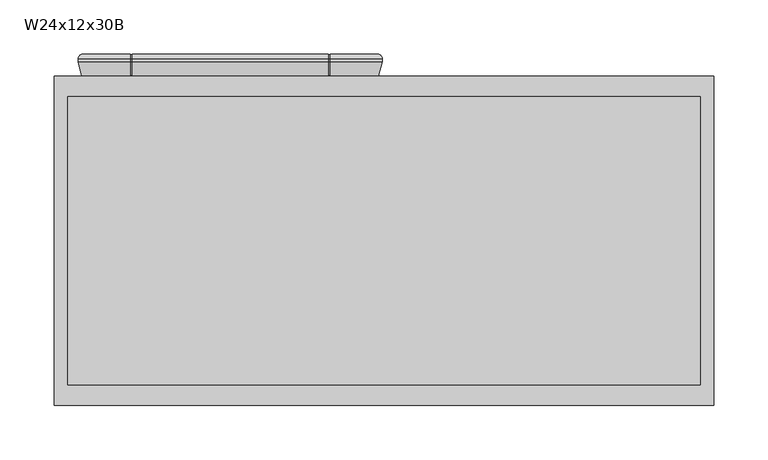
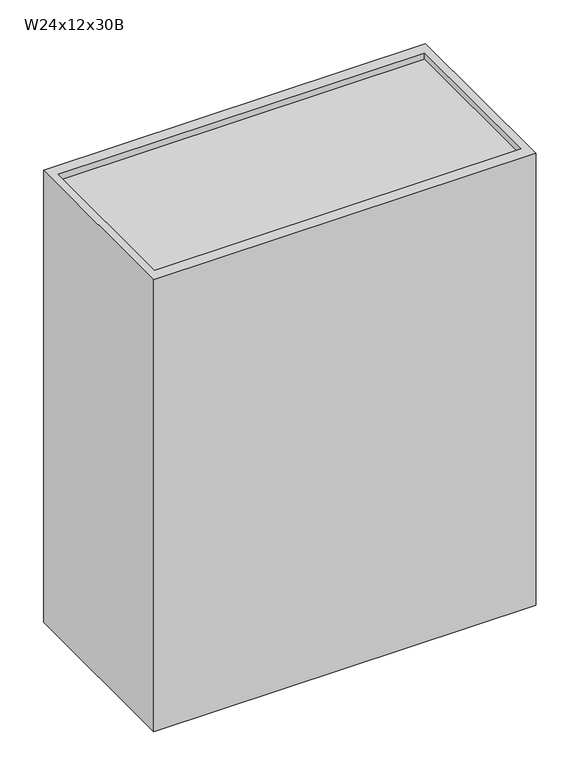
"""IFC4 building model written with IfcOpenShell, lengths in millimetres: furniture geometry, Cabinet-Wall-Merillat-Double_Door-Marlin : W24x12x30B."""

from ifc_helpers import new_model, si_unit, frame, origin, place, context, project, spatial, polyline, circle_curve, ellipse_curve, outline, extrude, faceted_brep, source, transform, mapped, element, save
from ifc_brep_helpers import plane_surface, cylinder_surface, advanced_brep


def w24x12x30b_f3964ec6(model_context):
    return source(origin(), model_context, "Body", "SolidModel", [
        advanced_brep(
        [(-24.0971608, 382.5621, 2108.2), (-21.0006683, 387.0325, 2105.1035075), (-21.0006683, 387.0325, 1400.0964925), (-24.0971608, 382.5621, 1397.0), (-24.0971608, 379.7935, 1397.0), (-24.0971608, 379.7935, 2108.2), (-20.5919608, 366.7125, 1400.5052), (-20.5919608, 366.7125, 2104.6948), (24.104002, 366.7125, 2059.9988372), (24.104002, 366.7125, 1445.2011628), (24.4741337, 367.50625, 1445.5712945), (26.5552927, 371.96931, 1447.6524535), (26.5552927, 371.96931, 2057.5475465), (24.4741337, 367.50625, 2059.6287055), (25.1555233, 374.2094093, 1446.252684), (25.1555233, 374.2094093, 2058.947316), (10.8278392, 374.4595, 1431.925), (10.8278392, 374.4595, 2073.275), (10.8278392, 379.2855, 1431.925), (10.8278392, 379.2855, 2073.275), (25.1555233, 379.5355907, 1446.252684), (25.1555233, 379.5355907, 2058.947316), (26.5552927, 381.77569, 1447.6524535), (26.5552927, 381.77569, 2057.5475465), (24.4741337, 386.23875, 1445.5712945), (24.1068694, 387.0263508, 1445.2040302), (24.104002, 387.0325, 2059.9988372), (24.4741337, 386.23875, 2059.6287055), (24.1068694, 387.0325, 1400.0964925), (24.1068694, 382.5621, 1397.0), (253.7938467, 387.0325, 1400.0964925), (256.8903392, 382.5621, 1397.0), (208.7261206, 382.5621, 1397.0), (208.7261206, 387.0325, 1400.0964925), (25.6943694, 382.5621, 1397.0), (25.6943694, 387.0325, 1400.0964925), (207.1386206, 387.0325, 1400.0964925), (207.1386206, 382.5621, 1397.0), (24.1068694, 379.7935, 1397.0), (256.8903392, 379.7935, 1397.0), (208.7261206, 379.7935, 1397.0), (25.6943694, 379.7935, 1397.0), (207.1386206, 379.7935, 1397.0), (24.1068694, 366.7125, 1400.5052), (253.3851392, 366.7125, 1400.5052), (208.7261206, 366.7125, 1400.5052), (25.6943694, 366.7125, 1400.5052), (207.1386206, 366.7125, 1400.5052), (206.2378857, 371.96931, 1447.6524535), (25.6943694, 367.50625, 1445.5712945), (25.6943694, 366.7125, 1445.2011628), (207.1386206, 366.7125, 1445.2011628), (207.1386206, 367.50625, 1445.5712945), (208.3190448, 367.50625, 1445.5712945), (207.6376552, 374.2094093, 1446.252684), (221.9653392, 374.4595, 1431.925), (221.9653392, 379.2855, 1431.925), (207.6376552, 379.5355907, 1446.252684), (206.2378857, 381.77569, 1447.6524535), (208.3190448, 386.23875, 1445.5712945), (207.1386206, 386.23875, 1445.5712945), (207.1386206, 387.0325, 1445.2011628), (25.6943694, 387.0325, 1445.2011628), (25.6943694, 386.23875, 1445.5712945), (253.7938467, 387.0325, 2105.1035075), (256.8903392, 382.5621, 2108.2), (256.8903392, 379.7935, 2108.2), (253.3851392, 366.7125, 2104.6948), (208.6891765, 366.7125, 1445.2011628), (208.6891765, 366.7125, 2059.9988372), (208.3190448, 367.50625, 2059.6287055), (206.2378857, 371.96931, 2057.5475465), (207.6376552, 374.2094093, 2058.947316), (221.9653392, 374.4595, 2073.275), (221.9653392, 379.2855, 2073.275), (207.6376552, 379.5355907, 2058.947316), (206.2378857, 381.77569, 2057.5475465), (208.3190448, 386.23875, 2059.6287055), (208.6891765, 387.0325, 2059.9988372), (208.6891765, 387.0325, 1445.2011628), (208.7261206, 387.0325, 2105.1035075), (208.7261206, 382.5621, 2108.2), (24.1068694, 382.5621, 2108.2), (24.1068694, 387.0325, 2105.1035075), (207.1386206, 382.5621, 2108.2), (207.1386206, 387.0325, 2105.1035075), (25.6943694, 387.0325, 2105.1035075), (25.6943694, 382.5621, 2108.2), (208.7261206, 379.7935, 2108.2), (24.1068694, 379.7935, 2108.2), (207.1386206, 379.7935, 2108.2), (25.6943694, 379.7935, 2108.2), (208.7261206, 366.7125, 2104.6948), (24.1068694, 366.7125, 2104.6948), (207.1386206, 366.7125, 2104.6948), (25.6943694, 366.7125, 2104.6948), (207.1386206, 366.7125, 2059.9988372), (25.6943694, 366.7125, 2059.9988372), (207.1386206, 367.50625, 2059.6287055), (25.6943694, 367.50625, 2059.6287055), (25.6943694, 386.23875, 2059.6287055), (25.6943694, 387.0325, 2059.9988372), (207.1386206, 387.0325, 2059.9988372), (207.1386206, 386.23875, 2059.6287055), (207.1386206, 367.50625, 2104.0857412), (207.1386206, 379.8980037, 2107.40625), (207.1386206, 382.5621, 2107.40625), (207.1386206, 386.23875, 2104.9526052), (208.7261206, 386.23875, 2059.6287055), (208.7261206, 386.23875, 2104.9526052), (208.7261206, 382.5621, 2107.40625), (208.7261206, 379.8980037, 2107.40625), (208.7261206, 367.50625, 2104.0857412), (208.7261206, 367.50625, 2059.6287055), (24.1068694, 367.50625, 2059.6287055), (24.1068694, 367.50625, 2104.0857412), (24.1068694, 379.8980037, 2107.40625), (24.1068694, 382.5621, 2107.40625), (24.1068694, 386.23875, 2104.9526052), (24.1068694, 386.23875, 2059.6287055), (25.6943694, 386.23875, 2104.9526052), (25.6943694, 382.5621, 2107.40625), (25.6943694, 379.8980037, 2107.40625), (25.6943694, 367.50625, 2104.0857412), (24.1068694, 386.23875, 1445.5712945), (24.1068694, 386.23875, 1400.2473948), (24.1068694, 382.5621, 1397.79375), (24.1068694, 379.8980037, 1397.79375), (24.1068694, 367.50625, 1401.1142588), (24.1068694, 367.50625, 1445.5712945), (25.6943694, 367.50625, 1401.1142588), (25.6943694, 379.8980037, 1397.79375), (25.6943694, 382.5621, 1397.79375), (25.6943694, 386.23875, 1400.2473948), (207.1386206, 386.23875, 1400.2473948), (207.1386206, 382.5621, 1397.79375), (207.1386206, 379.8980037, 1397.79375), (207.1386206, 367.50625, 1401.1142588), (208.7261206, 386.23875, 1445.5712945), (208.7261206, 367.50625, 1445.5712945), (208.7261206, 367.50625, 1401.1142588), (208.7261206, 379.8980037, 1397.79375), (208.7261206, 382.5621, 1397.79375), (208.7261206, 386.23875, 1400.2473948)],
        [
            (0, 1, ellipse_curve(frame((-19.3219608, 382.5621, 2103.4248), z_axis=(-0.7071067811865475, 0.0, -0.7071067811865475), x_axis=(-0.7071067811865474, 0.0, 0.7071067811865476)), 6.7531526, 4.7752)),
            (1, 2),
            (2, 3, ellipse_curve(frame((-19.3219608, 382.5621, 1401.7752), z_axis=(-0.7071067811865475, 0.0, 0.7071067811865475), x_axis=(0.7071067811865474, 0.0, 0.7071067811865476)), 6.7531526, 4.7752)),
            (3, 0),
            (3, 4),
            (4, 5),
            (5, 0),
            (4, 6),
            (6, 7),
            (7, 5),
            (8, 9),
            (9, 10),
            (10, 11),
            (11, 12),
            (12, 13),
            (13, 8),
            (11, 14, ellipse_curve(frame((25.1280392, 372.6348492, 1446.2252), z_axis=(-0.7071067811865475, 0.0, 0.7071067811865475), x_axis=(0.7071067811865474, 0.0, 0.7071067811865476)), 2.2271035, 1.5748)),
            (14, 15),
            (15, 12, ellipse_curve(frame((25.1280392, 372.6348492, 2058.9748), z_axis=(-0.7071067811865475, 0.0, -0.7071067811865475), x_axis=(-0.7071067811865474, 0.0, 0.7071067811865476)), 2.2271035, 1.5748)),
            (14, 16),
            (16, 17),
            (17, 15),
            (16, 18),
            (18, 19),
            (19, 17),
            (18, 20),
            (20, 21),
            (21, 19),
            (20, 22, ellipse_curve(frame((25.1280392, 381.1101508, 1446.2252), z_axis=(-0.7071067811865475, 0.0, 0.7071067811865475), x_axis=(0.7071067811865474, 0.0, 0.7071067811865476)), 2.2271035, 1.5748)),
            (22, 23),
            (23, 21, ellipse_curve(frame((25.1280392, 381.1101508, 2058.9748), z_axis=(-0.7071067811865475, 0.0, -0.7071067811865475), x_axis=(-0.7071067811865474, 0.0, 0.7071067811865476)), 2.2271035, 1.5748)),
            (22, 24),
            (24, 25),
            (25, 26),
            (26, 27),
            (27, 23),
            (2, 28),
            (28, 29, circle_curve(frame((24.1068694, 382.5621, 1401.7752), z_axis=(-1.0, 0.0, 0.0), x_axis=(0.0, -1.0, 0.0)), 4.7752)),
            (29, 3),
            (30, 31, ellipse_curve(frame((252.1151392, 382.5621, 1401.7752), z_axis=(-0.7071067811865475, 0.0, -0.7071067811865475), x_axis=(-0.7071067811865476, 0.0, 0.7071067811865474)), 6.7531526, 4.7752)),
            (31, 32),
            (32, 33, circle_curve(frame((208.7261206, 382.5621, 1401.7752), z_axis=(1.0, 0.0, 0.0), x_axis=(0.0, -1.0, 0.0)), 4.7752)),
            (33, 30),
            (34, 35, circle_curve(frame((25.6943694, 382.5621, 1401.7752), z_axis=(1.0, 0.0, 0.0), x_axis=(0.0, -1.0, 0.0)), 4.7752)),
            (35, 36),
            (36, 37, circle_curve(frame((207.1386206, 382.5621, 1401.7752), z_axis=(-1.0, 0.0, 0.0), x_axis=(0.0, -1.0, 0.0)), 4.7752)),
            (37, 34),
            (29, 38),
            (38, 4),
            (31, 39),
            (39, 40),
            (40, 32),
            (41, 34),
            (37, 42),
            (42, 41),
            (38, 43),
            (43, 6),
            (39, 44),
            (44, 45),
            (45, 40),
            (46, 41),
            (42, 47),
            (47, 46),
            (48, 11),
            (10, 49),
            (49, 50),
            (50, 51),
            (51, 52),
            (52, 53),
            (53, 48),
            (48, 54, ellipse_curve(frame((207.6651392, 372.6348492, 1446.2252), z_axis=(-0.7071067811865475, 0.0, -0.7071067811865475), x_axis=(-0.7071067811865476, 0.0, 0.7071067811865474)), 2.2271035, 1.5748)),
            (54, 14),
            (54, 55),
            (55, 16),
            (55, 56),
            (56, 18),
            (56, 57),
            (57, 20),
            (57, 58, ellipse_curve(frame((207.6651392, 381.1101508, 1446.2252), z_axis=(-0.7071067811865475, 0.0, -0.7071067811865475), x_axis=(-0.7071067811865476, 0.0, 0.7071067811865474)), 2.2271035, 1.5748)),
            (58, 22),
            (58, 59),
            (59, 60),
            (60, 61),
            (61, 62),
            (62, 63),
            (63, 24),
            (30, 64),
            (64, 65, ellipse_curve(frame((252.1151392, 382.5621, 2103.4248), z_axis=(0.7071067811865475, 0.0, -0.7071067811865475), x_axis=(-0.7071067811865474, 0.0, -0.7071067811865476)), 6.7531526, 4.7752)),
            (65, 31),
            (65, 66),
            (66, 39),
            (66, 67),
            (67, 44),
            (68, 69),
            (69, 70),
            (70, 71),
            (71, 48),
            (53, 68),
            (71, 72, ellipse_curve(frame((207.6651392, 372.6348492, 2058.9748), z_axis=(0.7071067811865475, 0.0, -0.7071067811865475), x_axis=(-0.7071067811865474, 0.0, -0.7071067811865476)), 2.2271035, 1.5748)),
            (72, 54),
            (72, 73),
            (73, 55),
            (73, 74),
            (74, 56),
            (74, 75),
            (75, 57),
            (75, 76, ellipse_curve(frame((207.6651392, 381.1101508, 2058.9748), z_axis=(0.7071067811865475, 0.0, -0.7071067811865475), x_axis=(-0.7071067811865474, 0.0, -0.7071067811865476)), 2.2271035, 1.5748)),
            (76, 58),
            (76, 77),
            (77, 78),
            (78, 79),
            (79, 59),
            (64, 80),
            (80, 81, circle_curve(frame((208.7261206, 382.5621, 2103.4248), z_axis=(1.0, 0.0, 0.0), x_axis=(0.0, -1.0, 0.0)), 4.7752)),
            (81, 65),
            (0, 82),
            (82, 83, circle_curve(frame((24.1068694, 382.5621, 2103.4248), z_axis=(-1.0, 0.0, 0.0), x_axis=(0.0, -1.0, 0.0)), 4.7752)),
            (83, 1),
            (84, 85, circle_curve(frame((207.1386206, 382.5621, 2103.4248), z_axis=(-1.0, 0.0, 0.0), x_axis=(0.0, -1.0, 0.0)), 4.7752)),
            (85, 86),
            (86, 87, circle_curve(frame((25.6943694, 382.5621, 2103.4248), z_axis=(1.0, 0.0, 0.0), x_axis=(0.0, -1.0, 0.0)), 4.7752)),
            (87, 84),
            (81, 88),
            (88, 66),
            (5, 89),
            (89, 82),
            (90, 84),
            (87, 91),
            (91, 90),
            (88, 92),
            (92, 67),
            (7, 93),
            (93, 89),
            (94, 90),
            (91, 95),
            (95, 94),
            (43, 9),
            (8, 93),
            (92, 69),
            (68, 45),
            (96, 94),
            (95, 97),
            (97, 96),
            (50, 46),
            (47, 51),
            (12, 71),
            (70, 98),
            (98, 96),
            (97, 99),
            (99, 13),
            (15, 72),
            (17, 73),
            (19, 74),
            (21, 75),
            (23, 76),
            (27, 100),
            (100, 101),
            (101, 102),
            (102, 103),
            (103, 77),
            (83, 26),
            (25, 28),
            (33, 79),
            (78, 80),
            (85, 102),
            (101, 86),
            (35, 62),
            (61, 36),
            (98, 104),
            (104, 105),
            (105, 106),
            (106, 107, circle_curve(frame((207.1386206, 382.5621, 2103.4248), z_axis=(-1.0, 0.0, 0.0), x_axis=(0.0, 0.0, 1.0)), 3.98145)),
            (107, 103),
            (78, 108),
            (108, 109),
            (109, 110, circle_curve(frame((208.7261206, 382.5621, 2103.4248), z_axis=(1.0, 0.0, 0.0), x_axis=(0.0, 0.0, 1.0)), 3.98145)),
            (110, 111),
            (111, 112),
            (112, 113),
            (113, 69),
            (77, 108),
            (107, 109),
            (106, 110),
            (105, 111),
            (104, 112),
            (70, 113),
            (8, 114),
            (114, 115),
            (115, 116),
            (116, 117),
            (117, 118, circle_curve(frame((24.1068694, 382.5621, 2103.4248), z_axis=(-1.0, 0.0, 0.0), x_axis=(0.0, 0.0, 1.0)), 3.98145)),
            (118, 119),
            (119, 26),
            (100, 120),
            (120, 121, circle_curve(frame((25.6943694, 382.5621, 2103.4248), z_axis=(1.0, 0.0, 0.0), x_axis=(0.0, 0.0, 1.0)), 3.98145)),
            (121, 122),
            (122, 123),
            (123, 99),
            (119, 27),
            (118, 120),
            (117, 121),
            (116, 122),
            (115, 123),
            (114, 13),
            (25, 124),
            (124, 125),
            (125, 126, circle_curve(frame((24.1068694, 382.5621, 1401.7752), z_axis=(-1.0, 0.0, 0.0), x_axis=(0.0, 0.0, 1.0)), 3.98145)),
            (126, 127),
            (127, 128),
            (128, 129),
            (129, 9),
            (49, 130),
            (130, 131),
            (131, 132),
            (132, 133, circle_curve(frame((25.6943694, 382.5621, 1401.7752), z_axis=(1.0, 0.0, 0.0), x_axis=(0.0, 0.0, 1.0)), 3.98145)),
            (133, 63),
            (129, 10),
            (128, 130),
            (127, 131),
            (126, 132),
            (125, 133),
            (124, 24),
            (60, 134),
            (134, 135, circle_curve(frame((207.1386206, 382.5621, 1401.7752), z_axis=(-1.0, 0.0, 0.0), x_axis=(0.0, 0.0, 1.0)), 3.98145)),
            (135, 136),
            (136, 137),
            (137, 52),
            (138, 79),
            (68, 139),
            (139, 140),
            (140, 141),
            (141, 142),
            (142, 143, circle_curve(frame((208.7261206, 382.5621, 1401.7752), z_axis=(1.0, 0.0, 0.0), x_axis=(0.0, 0.0, 1.0)), 3.98145)),
            (143, 138),
            (138, 59),
            (53, 139),
            (137, 140),
            (136, 141),
            (135, 142),
            (134, 143),
        ],
        [
            cylinder_surface(frame((-19.3219608, 382.5621, 2108.2), z_axis=(0.0, 0.0, 1.0), x_axis=(0.0, -1.0, 0.0)), 4.7752),
            plane_surface(frame((-24.0971608, 382.5621, 2108.2), z_axis=(-1.0, 0.0, 0.0), x_axis=(0.0, 0.0, -1.0))),
            plane_surface(frame((-24.0971608, 379.7935, 2108.2), z_axis=(-0.9659229350723619, -0.25882983502910506, 0.0), x_axis=(0.0, 0.0, -1.0))),
            plane_surface(frame((24.104002, 366.7125, 2059.9988372), z_axis=(0.9063077870366099, -0.4226182617407856, 0.0), x_axis=(0.0, 0.0, -1.0))),
            cylinder_surface(frame((25.1280392, 372.6348492, 2108.2), z_axis=(0.0, 0.0, 1.0000000000000002), x_axis=(0.01745240643729364, 0.9998476951563912, 0.0)), 1.5748),
            plane_surface(frame((25.1555233, 374.2094093, 2058.947316), z_axis=(0.017452406437322144, 0.9998476951563906, 0.0), x_axis=(0.0, 0.0, -1.0))),
            plane_surface(frame((10.8278392, 374.4595, 2073.275), z_axis=(1.0, 0.0, 0.0), x_axis=(0.0, 0.0, -1.0))),
            plane_surface(frame((10.8278392, 379.2855, 2073.275), z_axis=(0.01745240643727848, -0.9998476951563914, 0.0), x_axis=(0.0, 0.0, -1.0))),
            cylinder_surface(frame((25.1280392, 381.1101508, 2108.2), z_axis=(0.0, 0.0, 1.0000000000000002), x_axis=(0.9063077870367326, 0.42261826174052236, 0.0)), 1.5748),
            plane_surface(frame((26.5552927, 381.77569, 2057.5475465), z_axis=(0.9063077870366333, 0.4226182617407352, 0.0), x_axis=(0.0, 0.0, -1.0))),
            cylinder_surface(frame((-24.0971608, 382.5621, 1401.7752), z_axis=(-1.0, 0.0, 0.0), x_axis=(0.0, -1.0, 0.0)), 4.7752),
            plane_surface(frame((-24.0971608, 382.5621, 1397.0), z_axis=(0.0, 0.0, -1.0), x_axis=(1.0, 0.0, 0.0))),
            plane_surface(frame((-24.0971608, 379.7935, 1397.0), z_axis=(0.0, -0.2588298350291095, -0.9659229350723607), x_axis=(1.0, 0.0, 0.0))),
            plane_surface(frame((24.104002, 366.7125, 1445.2011628), z_axis=(0.0, -0.42261826174078143, 0.9063077870366119), x_axis=(1.0, 0.0, 0.0))),
            cylinder_surface(frame((-24.0971608, 372.6348492, 1446.2252), z_axis=(-1.0000000000000002, 0.0, 0.0), x_axis=(0.0, 0.9998476951563913, 0.017452406437289025)), 1.5748),
            plane_surface(frame((25.1555233, 374.2094093, 1446.252684), z_axis=(0.0, 0.9998476951563907, 0.01745240643731753), x_axis=(1.0, 0.0, 0.0))),
            plane_surface(frame((10.8278392, 374.4595, 1431.925), z_axis=(0.0, 0.0, 1.0), x_axis=(1.0, 0.0, 0.0))),
            plane_surface(frame((10.8278392, 379.2855, 1431.925), z_axis=(0.0, -0.9998476951563913, 0.017452406437283095), x_axis=(1.0, 0.0, 0.0))),
            cylinder_surface(frame((-24.0971608, 381.1101508, 1446.2252), z_axis=(-1.0000000000000002, 0.0, 0.0), x_axis=(0.0, 0.4226182617405265, 0.9063077870367306)), 1.5748),
            plane_surface(frame((26.5552927, 381.77569, 1447.6524535), z_axis=(0.0, 0.4226182617407394, 0.9063077870366314), x_axis=(1.0, 0.0, 0.0))),
            cylinder_surface(frame((252.1151392, 382.5621, 1397.0), z_axis=(0.0, 0.0, -1.0), x_axis=(0.0, -1.0, 0.0)), 4.7752),
            plane_surface(frame((256.8903392, 382.5621, 1397.0), z_axis=(1.0, 0.0, 0.0), x_axis=(0.0, 0.0, 1.0))),
            plane_surface(frame((256.8903392, 379.7935, 1397.0), z_axis=(0.9659229350723619, -0.25882983502910506, 0.0), x_axis=(0.0, 0.0, 1.0))),
            plane_surface(frame((208.6891765, 366.7125, 1445.2011628), z_axis=(-0.9063077870366099, -0.4226182617407856, 0.0), x_axis=(0.0, 0.0, 1.0))),
            cylinder_surface(frame((207.6651392, 372.6348492, 1397.0), z_axis=(0.0, 0.0, -1.0000000000000002), x_axis=(-0.01745240643729364, 0.9998476951563912, 0.0)), 1.5748),
            plane_surface(frame((207.6376552, 374.2094093, 1446.252684), z_axis=(-0.017452406437322144, 0.9998476951563906, 0.0), x_axis=(0.0, 0.0, 1.0))),
            plane_surface(frame((221.9653392, 374.4595, 1431.925), z_axis=(-1.0, 0.0, 0.0), x_axis=(0.0, 0.0, 1.0))),
            plane_surface(frame((221.9653392, 379.2855, 1431.925), z_axis=(-0.01745240643727848, -0.9998476951563914, 0.0), x_axis=(0.0, 0.0, 1.0))),
            cylinder_surface(frame((207.6651392, 381.1101508, 1397.0), z_axis=(0.0, 0.0, -1.0000000000000002), x_axis=(-0.9063077870367326, 0.42261826174052236, 0.0)), 1.5748),
            plane_surface(frame((206.2378857, 381.77569, 1447.6524535), z_axis=(-0.9063077870366333, 0.4226182617407352, 0.0), x_axis=(0.0, 0.0, 1.0))),
            cylinder_surface(frame((256.8903392, 382.5621, 2103.4248), z_axis=(1.0, 0.0, 0.0), x_axis=(0.0, -1.0, 0.0)), 4.7752),
            plane_surface(frame((256.8903392, 382.5621, 2108.2), z_axis=(0.0, 0.0, 1.0), x_axis=(-1.0, 0.0, 0.0))),
            plane_surface(frame((256.8903392, 379.7935, 2108.2), z_axis=(0.0, -0.2588298350291006, 0.9659229350723632), x_axis=(-1.0, 0.0, 0.0))),
            plane_surface(frame((253.3851392, 366.7125, 2104.6948), z_axis=(0.0, -1.0, 0.0), x_axis=(-1.0, 0.0, 0.0))),
            plane_surface(frame((208.6891765, 366.7125, 2059.9988372), z_axis=(0.0, -0.42261826174078976, -0.9063077870366079), x_axis=(-1.0, 0.0, 0.0))),
            cylinder_surface(frame((256.8903392, 372.6348492, 2058.9748), z_axis=(1.0000000000000002, 0.0, 0.0), x_axis=(0.0, 0.999847695156391, -0.017452406437298253)), 1.5748),
            plane_surface(frame((207.6376552, 374.2094093, 2058.947316), z_axis=(0.0, 0.9998476951563905, -0.01745240643732676), x_axis=(-1.0, 0.0, 0.0))),
            plane_surface(frame((221.9653392, 374.4595, 2073.275), z_axis=(0.0, 0.0, -1.0), x_axis=(-1.0, 0.0, 0.0))),
            plane_surface(frame((221.9653392, 379.2855, 2073.275), z_axis=(0.0, -0.9998476951563915, -0.017452406437273867), x_axis=(-1.0, 0.0, 0.0))),
            cylinder_surface(frame((256.8903392, 381.1101508, 2058.9748), z_axis=(1.0000000000000002, 0.0, 0.0), x_axis=(0.0, 0.4226182617405182, -0.9063077870367346)), 1.5748),
            plane_surface(frame((206.2378857, 381.77569, 2057.5475465), z_axis=(0.0, 0.422618261740731, -0.9063077870366353), x_axis=(-1.0, 0.0, 0.0))),
            plane_surface(frame((208.6891765, 387.0325, 2059.9988372), z_axis=(0.0, 1.0, 0.0), x_axis=(-1.0, 0.0, 0.0))),
            plane_surface(frame((207.1386206, 387.0325, 2059.9988372), z_axis=(1.0000000000000002, 0.0, 0.0), x_axis=(0.0, -0.9063077870366335, -0.422618261740735))),
            plane_surface(frame((208.7261206, 387.0325, 2059.9988372), z_axis=(-1.0000000000000002, 0.0, 0.0), x_axis=(0.0, 0.9063077870366335, 0.422618261740735))),
            plane_surface(frame((207.1386206, 387.0325, 2059.9988372), z_axis=(0.0, -0.422618261740735, 0.9063077870366335), x_axis=(1.0, 0.0, 0.0))),
            plane_surface(frame((207.1386206, 386.23875, 2059.6287055), z_axis=(0.0, 1.0, 0.0), x_axis=(1.0, 0.0, 0.0))),
            cylinder_surface(frame((208.7261206, 382.5621, 2103.4248), z_axis=(1.0, 0.0, 0.0), x_axis=(0.0, 0.0, 1.0)), 3.98145),
            plane_surface(frame((207.1386206, 382.5621, 2107.40625), z_axis=(0.0, 0.0, 1.0), x_axis=(1.0, 0.0, 0.0))),
            plane_surface(frame((207.1386206, 379.8980037, 2107.40625), z_axis=(0.0, -0.2588298350291711, 0.9659229350723443), x_axis=(1.0, 0.0, 0.0))),
            plane_surface(frame((207.1386206, 367.50625, 2104.0857412), z_axis=(0.0, -1.0, 0.0), x_axis=(1.0, 0.0, 0.0))),
            plane_surface(frame((207.1386206, 367.50625, 2059.6287055), z_axis=(0.0, 0.4226182617408151, 0.906307787036596), x_axis=(1.0, 0.0, 0.0))),
            plane_surface(frame((24.1068694, 387.0325, 2059.9988372), z_axis=(1.0000000000000002, 0.0, 0.0), x_axis=(0.0, -0.9063077870366413, -0.42261826174071837))),
            plane_surface(frame((25.6943694, 387.0325, 2059.9988372), z_axis=(-1.0000000000000002, 0.0, 0.0), x_axis=(0.0, 0.9063077870366413, 0.42261826174071837))),
            plane_surface(frame((24.1068694, 387.0325, 2059.9988372), z_axis=(0.0, -0.42261826174071837, 0.9063077870366413), x_axis=(1.0, 0.0, 0.0))),
            plane_surface(frame((24.1068694, 386.23875, 2059.6287055), z_axis=(0.0, 1.0, 0.0), x_axis=(1.0, 0.0, 0.0))),
            cylinder_surface(frame((25.6943694, 382.5621, 2103.4248), z_axis=(1.0, 0.0, 0.0), x_axis=(0.0, 0.0, 1.0)), 3.98145),
            plane_surface(frame((24.1068694, 382.5621, 2107.40625), z_axis=(0.0, 0.0, 1.0), x_axis=(1.0, 0.0, 0.0))),
            plane_surface(frame((24.1068694, 379.8980037, 2107.40625), z_axis=(0.0, -0.2588298350291734, 0.9659229350723437), x_axis=(1.0, 0.0, 0.0))),
            plane_surface(frame((24.1068694, 367.50625, 2104.0857412), z_axis=(0.0, -1.0, 0.0), x_axis=(1.0, 0.0, 0.0))),
            plane_surface(frame((24.1068694, 367.50625, 2059.6287055), z_axis=(0.0, 0.4226182617408322, 0.9063077870365881), x_axis=(1.0, 0.0, 0.0))),
            plane_surface(frame((24.1068694, 382.5621, 1406.5504), z_axis=(1.0, 0.0, 0.0), x_axis=(0.0, 1.0, 0.0))),
            plane_surface(frame((25.6943694, 382.5621, 1406.5504), z_axis=(-1.0, 0.0, 0.0), x_axis=(0.0, -1.0, 0.0))),
            plane_surface(frame((24.1068694, 366.7125, 1445.2011628), z_axis=(0.0, 0.4226182617408193, -0.906307787036594), x_axis=(1.0, 0.0, 0.0))),
            plane_surface(frame((24.1068694, 367.50625, 1445.5712945), z_axis=(0.0, -1.0, 0.0), x_axis=(1.0, 0.0, 0.0))),
            plane_surface(frame((24.1068694, 367.50625, 1401.1142588), z_axis=(0.0, -0.258829835029436, -0.9659229350722732), x_axis=(1.0, 0.0, 0.0))),
            plane_surface(frame((24.1068694, 379.8980037, 1397.79375), z_axis=(0.0, 0.0, -1.0), x_axis=(1.0, 0.0, 0.0))),
            cylinder_surface(frame((25.6943694, 382.5621, 1401.7752), z_axis=(1.0, 0.0, 0.0), x_axis=(0.0, 0.0, 1.0)), 3.98145),
            plane_surface(frame((24.1068694, 386.23875, 1400.2473948), z_axis=(0.0, 1.0, 0.0), x_axis=(1.0, 0.0, 0.0))),
            plane_surface(frame((24.1068694, 386.23875, 1445.5712945), z_axis=(0.0, -0.42261826174073513, -0.9063077870366334), x_axis=(1.0, 0.0, 0.0))),
            plane_surface(frame((207.1386206, 386.23875, 1445.5712945), z_axis=(1.0, 0.0, 0.0), x_axis=(0.0, 0.9063077870366235, -0.4226182617407563))),
            plane_surface(frame((208.7261206, 386.23875, 1445.5712945), z_axis=(-1.0, 0.0, 0.0), x_axis=(0.0, -0.9063077870366235, 0.4226182617407563))),
            plane_surface(frame((207.1386206, 386.23875, 1445.5712945), z_axis=(0.0, -0.4226182617407563, -0.9063077870366235), x_axis=(1.0, 0.0, 0.0))),
            plane_surface(frame((207.1386206, 366.7125, 1445.2011628), z_axis=(0.0, 0.42261826174079387, -0.9063077870366061), x_axis=(1.0, 0.0, 0.0))),
            plane_surface(frame((207.1386206, 367.50625, 1445.5712945), z_axis=(0.0, -1.0, 0.0), x_axis=(1.0, 0.0, 0.0))),
            plane_surface(frame((207.1386206, 367.50625, 1401.1142588), z_axis=(0.0, -0.258829835029439, -0.9659229350722724), x_axis=(1.0, 0.0, 0.0))),
            plane_surface(frame((207.1386206, 379.8980037, 1397.79375), z_axis=(0.0, 0.0, -1.0), x_axis=(1.0, 0.0, 0.0))),
            cylinder_surface(frame((208.7261206, 382.5621, 1401.7752), z_axis=(1.0, 0.0, 0.0), x_axis=(0.0, 0.0, 1.0)), 3.98145),
            plane_surface(frame((207.1386206, 386.23875, 1400.2473948), z_axis=(0.0, 1.0, 0.0), x_axis=(1.0, 0.0, 0.0))),
        ],
        [
            (0, [[1, 2, 3, 4]]),
            (1, [[-4, 5, 6, 7]]),
            (2, [[-6, 8, 9, 10]]),
            (3, [[11, 12, 13, 14, 15, 16]]),
            (4, [[-14, 17, 18, 19]]),
            (5, [[-18, 20, 21, 22]]),
            (6, [[-21, 23, 24, 25]]),
            (7, [[-24, 26, 27, 28]]),
            (8, [[-27, 29, 30, 31]]),
            (9, [[-30, 32, 33, 34, 35, 36]]),
            (10, [[-3, 37, 38, 39]]),
            (10, [[40, 41, 42, 43]]),
            (10, [[44, 45, 46, 47]]),
            (11, [[-5, -39, 48, 49]]),
            (11, [[50, 51, 52, -41]]),
            (11, [[53, -47, 54, 55]]),
            (12, [[-8, -49, 56, 57]]),
            (12, [[58, 59, 60, -51]]),
            (12, [[61, -55, 62, 63]]),
            (13, [[64, -13, 65, 66, 67, 68, 69, 70]]),
            (14, [[-17, -64, 71, 72]]),
            (15, [[-20, -72, 73, 74]]),
            (16, [[-23, -74, 75, 76]]),
            (17, [[-26, -76, 77, 78]]),
            (18, [[-29, -78, 79, 80]]),
            (19, [[-80, 81, 82, 83, 84, 85, 86, -32]]),
            (20, [[-40, 87, 88, 89]]),
            (21, [[-50, -89, 90, 91]]),
            (22, [[-58, -91, 92, 93]]),
            (23, [[94, 95, 96, 97, -70, 98]]),
            (24, [[-71, -97, 99, 100]]),
            (25, [[-73, -100, 101, 102]]),
            (26, [[-75, -102, 103, 104]]),
            (27, [[-77, -104, 105, 106]]),
            (28, [[-79, -106, 107, 108]]),
            (29, [[-108, 109, 110, 111, 112, -81]]),
            (30, [[-88, 113, 114, 115]]),
            (30, [[-1, 116, 117, 118]]),
            (30, [[119, 120, 121, 122]]),
            (31, [[-90, -115, 123, 124]]),
            (31, [[-7, 125, 126, -116]]),
            (31, [[127, -122, 128, 129]]),
            (32, [[-92, -124, 130, 131]]),
            (32, [[-10, 132, 133, -125]]),
            (32, [[134, -129, 135, 136]]),
            (33, [[-9, -57, 137, -11, 138, -132]]),
            (33, [[-93, -131, 139, -94, 140, -59]]),
            (33, [[141, -136, 142, 143]]),
            (33, [[144, -63, 145, -67]]),
            (34, [[146, -96, 147, 148, -143, 149, 150, -15]]),
            (35, [[-19, 151, -99, -146]]),
            (36, [[-22, 152, -101, -151]]),
            (37, [[-25, 153, -103, -152]]),
            (38, [[-28, 154, -105, -153]]),
            (39, [[-31, 155, -107, -154]]),
            (40, [[-155, -36, 156, 157, 158, 159, 160, -109]]),
            (41, [[-2, -118, 161, -34, 162, -37]]),
            (41, [[-87, -43, 163, -111, 164, -113]]),
            (41, [[165, -158, 166, -120]]),
            (41, [[167, -84, 168, -45]]),
            (42, [[169, 170, 171, 172, 173, -159, -165, -119, -127, -134, -141, -148]]),
            (43, [[174, 175, 176, 177, 178, 179, 180, -139, -130, -123, -114, -164]]),
            (44, [[-174, -110, 181]]),
            (45, [[-173, 182, -175, -181, -160]]),
            (46, [[-172, 183, -176, -182]]),
            (47, [[-171, 184, -177, -183]]),
            (48, [[-170, 185, -178, -184]]),
            (49, [[-169, -147, 186, -179, -185]]),
            (50, [[-180, -186, -95]]),
            (51, [[187, 188, 189, 190, 191, 192, 193, -161, -117, -126, -133, -138]]),
            (52, [[194, 195, 196, 197, 198, -149, -142, -135, -128, -121, -166, -157]]),
            (53, [[-193, 199, -35]]),
            (54, [[-192, 200, -194, -156, -199]]),
            (55, [[-191, 201, -195, -200]]),
            (56, [[-190, 202, -196, -201]]),
            (57, [[-189, 203, -197, -202]]),
            (58, [[-188, 204, -150, -198, -203]]),
            (59, [[-187, -16, -204]]),
            (60, [[205, 206, 207, 208, 209, 210, 211, -137, -56, -48, -38, -162]]),
            (61, [[212, 213, 214, 215, 216, -85, -167, -44, -53, -61, -144, -66]]),
            (62, [[-211, 217, -12]]),
            (63, [[-210, 218, -212, -65, -217]]),
            (64, [[-209, 219, -213, -218]]),
            (65, [[-208, 220, -214, -219]]),
            (66, [[-207, 221, -215, -220]]),
            (67, [[-206, 222, -86, -216, -221]]),
            (68, [[-205, -33, -222]]),
            (69, [[223, 224, 225, 226, 227, -68, -145, -62, -54, -46, -168, -83]]),
            (70, [[228, -163, -42, -52, -60, -140, 229, 230, 231, 232, 233, 234]]),
            (71, [[-228, 235, -112]]),
            (72, [[-229, -98, 236]]),
            (73, [[-227, 237, -230, -236, -69]]),
            (74, [[-226, 238, -231, -237]]),
            (75, [[-225, 239, -232, -238]]),
            (76, [[-224, 240, -233, -239]]),
            (77, [[-223, -82, -235, -234, -240]]),
        ],
    ),
        extrude(outline(polyline([(221.9653392, 379.2855), (221.9653392, 374.4595), (10.8278392, 374.4595), (10.8278392, 379.2855), (221.9653392, 379.2855)])), frame((0.0, 0.0, 1431.925), z_axis=(0.0, 0.0, 1.0), x_axis=(1.0, 0.0, 0.0)), (0.0, 0.0, 1.0), 641.35),
        extrude(outline(polyline([(-8.5711577, 347.6625), (525.0128185, 347.6625), (525.0128185, 80.9625), (-8.5711577, 80.9625), (-8.5711577, 347.6625)])), frame((0.0, 0.0, 1952.625), z_axis=(0.0, 0.0, 1.0), x_axis=(1.0, 0.0, 0.0)), (0.0, 0.0, 1.0), 19.05),
        extrude(outline(polyline([(-8.5711577, 347.6625), (525.0128185, 347.6625), (525.0128185, 80.9625), (-8.5711577, 80.9625), (-8.5711577, 347.6625)])), frame((0.0, 0.0, 1533.525), z_axis=(0.0, 0.0, 1.0), x_axis=(1.0, 0.0, 0.0)), (0.0, 0.0, 1.0), 19.05),
        extrude(outline(polyline([(-8.5711577, 347.6625), (525.0128185, 347.6625), (525.0128185, 80.9625), (-8.5711577, 80.9625), (-8.5711577, 347.6625)])), frame((0.0, 0.0, 1743.075), z_axis=(0.0, 0.0, 1.0), x_axis=(1.0, 0.0, 0.0)), (0.0, 0.0, 1.0), 19.05),
        faceted_brep([(-46.3221608, 61.9125, 2133.6), (-46.3221608, 61.9125, 1371.6), (563.2778392, 61.9125, 1371.6), (563.2778392, 61.9125, 2133.6), (-46.3221608, 366.7125, 2133.6), (563.2778392, 366.7125, 2133.6), (563.2778392, 366.7125, 1371.6), (-46.3221608, 366.7125, 1371.6), (525.0128185, 366.7125, 2095.2735163), (301.9690685, 366.7125, 2095.2735163), (301.9690685, 366.7125, 1409.4672696), (525.0128185, 366.7125, 1409.4672696), (-8.5711577, 366.7125, 2095.2735163), (-8.5711577, 366.7125, 1409.4672696), (214.98661, 366.7125, 1409.4672696), (214.98661, 366.7125, 2095.2735163), (-33.6221608, 80.9625, 1371.6), (550.5778392, 80.9625, 1371.6), (550.5778392, 347.6625, 1371.6), (-33.6221608, 347.6625, 1371.6), (550.5778392, 347.6625, 2133.6), (550.5778392, 80.9625, 2133.6), (-33.6221608, 80.9625, 2133.6), (-33.6221608, 347.6625, 2133.6), (-8.5711577, 80.9625, 2095.2735163), (214.98661, 347.6625, 2095.2735163), (301.9690685, 347.6625, 2095.2735163), (525.0128185, 80.9625, 2095.2735163), (525.0128185, 80.9625, 1409.4672696), (301.9690685, 347.6625, 1409.4672696), (214.98661, 347.6625, 1409.4672696), (-8.5711577, 80.9625, 1409.4672696), (550.5778392, 80.9625, 2122.9851371), (550.5778392, 347.6625, 2122.9851371), (-33.6221608, 347.6625, 2122.9851371), (-33.6221608, 80.9625, 2122.9851371), (-33.6221608, 80.9625, 1381.4352657), (-33.6221608, 347.6625, 1381.4352657), (550.5778392, 347.6625, 1381.4352657), (550.5778392, 80.9625, 1381.4352657)], [[[0, 1, 2, 3]], [[4, 5, 6, 7], [8, 9, 10, 11], [12, 13, 14, 15]], [[1, 0, 4, 7]], [[2, 1, 7, 6], [16, 17, 18, 19]], [[3, 2, 6, 5]], [[0, 3, 5, 4], [20, 21, 22, 23]], [[24, 12, 15, 25, 26, 9, 8, 27]], [[8, 11, 28, 27]], [[28, 11, 10, 29, 30, 14, 13, 31]], [[13, 12, 24, 31]], [[32, 33, 34, 35]], [[33, 32, 21, 20]], [[34, 33, 20, 23]], [[35, 34, 23, 22]], [[32, 35, 22, 21]], [[36, 37, 38, 39]], [[36, 39, 17, 16]], [[39, 38, 18, 17]], [[38, 37, 19, 18]], [[37, 36, 16, 19]], [[24, 27, 28, 31]], [[26, 29, 10, 9]], [[15, 14, 30, 25]], [[29, 26, 25, 30]]]),
    ])


if __name__ == "__main__":
    model = new_model("IFC4")
    model_context = context("Model", 3, world=origin())
    ifc_project = project(units=[si_unit("LENGTHUNIT", "METRE", prefix="MILLI")], contexts=[model_context])
    site = spatial("IfcSite", under=ifc_project)
    building = spatial("IfcBuilding", under=site)
    placement = place(None, origin())
    w24x12x30b_shape = w24x12x30b_f3964ec6(model_context)
    element("IfcFurniture", 1, ObjectType="Cabinet-Wall-Merillat-Double_Door-Marlin : W24x12x30B", at=placement, inside=building, context=model_context, shape_type="MappedRepresentation", body=[
        mapped(w24x12x30b_shape, transform((0.0, 0.0, 0.0), x_axis=(1.0, 0.0, 0.0), y_axis=(0.0, 1.0, 0.0), z_axis=(0.0, 0.0, 1.0))),
    ])
    save(model, "model.ifc")

# Revit data of these elements
# Type "Cabinet-Wall-Merillat-Double_Door-Marlin : W24x12x30B"
#   URL = "https://www.merillat.com/"
#   Product Page URL = "https://www.merillat.com/our-products/"
#   Product Line = "Express"
#   Product Group = "Wall Cabinet"
#   Product Documentation Link = "http://merillatbusiness.com/wp-content/uploads/2014/07/Merillat_Classic_Catalog.pdf"
#   Model = "W2442B"
#   Manufacturer = "Merillat"
#   Height Note = "Actual Height of 21 inches Cabinet is 20 1/2 inches"
#   Glass Door Note = "Glass Cabinet doors are only available in specific sizes. Please refer to the catalog for this information before requesting a glass size."
#   Finish = "Wood"
#   Description = "Wall 2442 Butt Door"
#   Construction Type = "Wall Cabinet"
#   Cabinet Construction Note = "Cabinets with B suffix have BUTT doors without a center frame stile:"
#   Assembly Code = "C1030410"
#   Spacing = 0' - 1"
#   Shelving Height = 0' - 6 3/4"
#   Door Spacing = 0' - 0 1/8"
#   Cabinet Door Width = 0' - 11 1/16"
#   Cabinet Door Height = 2' - 4"
#   Depth = 1' - 0"
#   Height = 2' - 6"
#   Top Of Cabinet = 7' - 0"
#   Width = 2' - 0"
#   COBie.Type = no
#   Top and Bottom Visibility = yes
#   Partial Overlay Butt = yes
#   Partial Overlay = no
#   Number of Shelves Greater than one = 3
#   Number of Shelves = 3
#   Middle Shelf = yes
#   Full Overlay Butt = no
#   Full Overlay = no
#   Elevation Swing Line = yes
#   Door Drawer Material = Wood - Merillat - Pecan(1)
#   Cabinet Material = Wood - Merillat - Pecan(1)
#   Cabinet Door Style = element 806847
# Element 1 (IfcFurniture, "Cabinet-Wall-Merillat-Double_Door-Marlin : W24x12x30B")
#   Materials on its faces: "Wood - Merillat - Pecan(1)"
# Materials
#   "Wood - Merillat - Pecan(1)": class "Wood", colour RGB 108 67 43, transparency 0, Cost = 0
